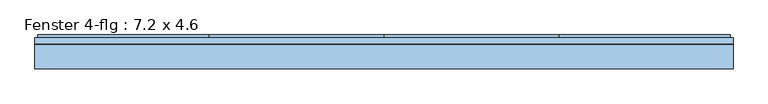
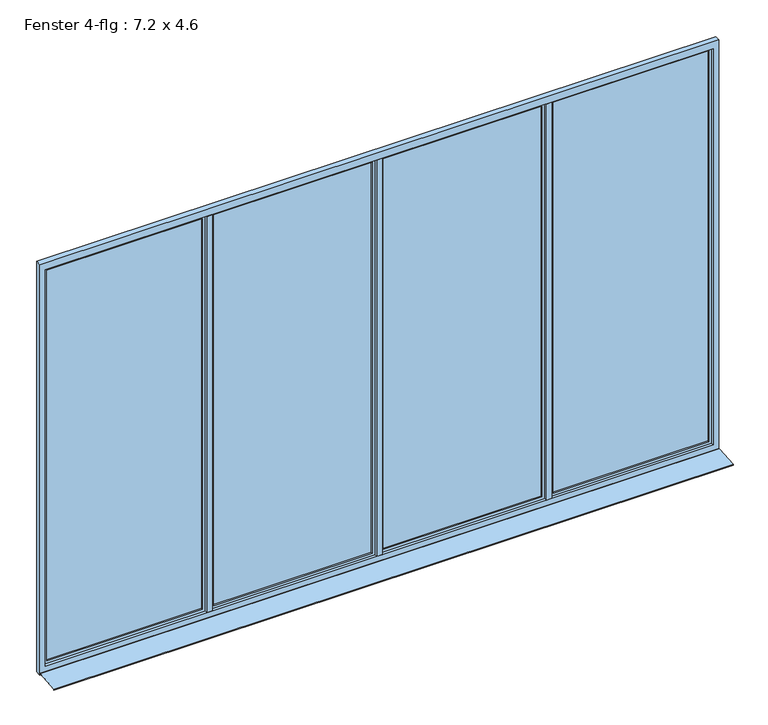
"""IFC4 building model written with IfcOpenShell, lengths in millimetres: window geometry, Fenster 4-flg : 7.2 x 4.6."""

import ifcopenshell
import ifcopenshell.guid

model = None  # the IFC model being written
_history = None  # IfcOwnerHistory: only IFC2X3 demands one
_inside = {}  # id of a spatial element -> (the spatial element, [elements in it])
_under = {}  # id of a project, library or spatial element -> (it, [spatial elements below it])
_declared = {}  # id of a project -> (the project, [libraries it declares])
_typed = {}  # id of a type object -> (the type object, [elements of that type])
_made_of = {}  # id of a material, layer set ... -> (it, [elements and type objects made of it])


def new_model(schema):
    """Start an empty IFC model of exactly this schema.

    Asked for "IFC4X3", IfcOpenShell would pick the latest addendum, in which some entities
    have other attributes; the version numbers below select the first issue.
    IFC2X3 requires an IfcOwnerHistory on every rooted entity: one is made here for all.
    """
    global model, _history
    if schema == "IFC4X3":
        model = ifcopenshell.file(schema_version=(4, 3, 0, 0))
    else:
        model = ifcopenshell.file(schema=schema)
    _inside.clear()
    _under.clear()
    _declared.clear()
    _typed.clear()
    _made_of.clear()
    _history = None
    if model.schema == "IFC2X3":
        org = make("IfcOrganization", Name="unknown")
        user = make(
            "IfcPersonAndOrganization",
            ThePerson=make("IfcPerson", FamilyName="unknown"),
            TheOrganization=org,
        )
        app = make(
            "IfcApplication",
            ApplicationDeveloper=org,
            Version="unknown",
            ApplicationFullName="unknown",
            ApplicationIdentifier="unknown",
        )
        _history = make(
            "IfcOwnerHistory",
            OwningUser=user,
            OwningApplication=app,
            ChangeAction="ADDED",
            CreationDate=0,
        )
    return model


def make(cls, **values):
    """One entity of the class cls with the attributes given. An attribute that is None is left unset."""
    return model.create_entity(
        cls, **{name: value for name, value in values.items() if value is not None}
    )


def rooted(cls, **values):
    """An entity with a GlobalId (a new one), such as an element, a storey or a relation."""
    return make(cls, GlobalId=ifcopenshell.guid.new(), OwnerHistory=_history, **values)


def si_unit(unit_type, name, prefix=None):
    """IfcSIUnit, for example si_unit("LENGTHUNIT", "METRE", prefix="MILLI")."""
    return make("IfcSIUnit", UnitType=unit_type, Prefix=prefix, Name=name)


def assignment(units):
    """IfcUnitAssignment: the units of a project."""
    return None if units is None else make("IfcUnitAssignment", Units=units)


def point(xyz):
    """IfcCartesianPoint."""
    return None if xyz is None else make("IfcCartesianPoint", Coordinates=xyz)


def direction(xyz):
    """IfcDirection."""
    return None if xyz is None else make("IfcDirection", DirectionRatios=xyz)


def frame(location, z_axis=None, x_axis=None):
    """IfcAxis2Placement3D, a coordinate frame: its origin and axes. An axis left out is left unset."""
    return make(
        "IfcAxis2Placement3D",
        Location=point(location),
        Axis=direction(z_axis),
        RefDirection=direction(x_axis),
    )


def origin():
    """The frame at (0, 0, 0) with its axes left unset."""
    return frame((0.0, 0.0, 0.0))


def place(relative_to, where):
    """IfcLocalPlacement: puts the frame where relative to a parent placement (None: the world)."""
    return make(
        "IfcLocalPlacement", PlacementRelTo=relative_to, RelativePlacement=where
    )


def context(
    kind, dimensions, precision=None, world=None, true_north=None, identifier=None
):
    """IfcGeometricRepresentationContext, for example the 3D "Model" context."""
    return make(
        "IfcGeometricRepresentationContext",
        ContextIdentifier=identifier,
        ContextType=kind,
        CoordinateSpaceDimension=dimensions,
        Precision=precision,
        WorldCoordinateSystem=world,
        TrueNorth=true_north,
    )


def project(units=None, contexts=None):
    """IfcProject with its units and contexts."""
    return rooted(
        "IfcProject",
        Name="project",
        RepresentationContexts=contexts,
        UnitsInContext=assignment(units),
    )


def spatial(cls, under=None, at=None, **own):
    """A site, building, storey or space (cls), placed at a placement, below another one or the project."""
    s = rooted(cls, ObjectPlacement=at, **own)
    if under is not None:
        _under.setdefault(under.id(), (under, []))[1].append(s)
    return s


def polyline(points):
    """IfcPolyline through the points."""
    return make("IfcPolyline", Points=[point(p) for p in points])


def outline(outer, holes=None, kind="AREA"):
    """IfcArbitraryClosedProfileDef: a profile drawn as a closed curve; with holes, ...WithVoids."""
    if holes is None:
        return make("IfcArbitraryClosedProfileDef", ProfileType=kind, OuterCurve=outer)
    return make(
        "IfcArbitraryProfileDefWithVoids",
        ProfileType=kind,
        OuterCurve=outer,
        InnerCurves=holes,
    )


def extrude(swept, where, along, depth):
    """IfcExtrudedAreaSolid: the profile swept, set in the frame where, extruded along a direction by depth."""
    return make(
        "IfcExtrudedAreaSolid",
        SweptArea=swept,
        Position=where,
        ExtrudedDirection=direction(along),
        Depth=depth,
    )


def faces_of(points, faces, orient=None, outer=None):
    """IfcFace entities. A face is a list of loops; a loop is a list of indices into points, from 0.

    orient and outer hold one flag for each loop. By default every Orientation is true, the
    first loop of a face is its IfcFaceOuterBound and the others are IfcFaceBound.
    """
    made = []
    for i, loops in enumerate(faces):
        bounds = []
        for j, loop in enumerate(loops):
            is_outer = j == 0 if outer is None else outer[i][j]
            bounds.append(
                make(
                    "IfcFaceOuterBound" if is_outer else "IfcFaceBound",
                    Bound=make("IfcPolyLoop", Polygon=[points[k] for k in loop]),
                    Orientation=True if orient is None else orient[i][j],
                )
            )
        made.append(make("IfcFace", Bounds=bounds))
    return made


def faceted_brep(points, faces, orient=None, outer=None, voids=None):
    """IfcFacetedBrep: a solid bounded by flat faces; with voids (closed shells), ...WithVoids."""
    shared = [point(p) for p in points]
    hull = make("IfcClosedShell", CfsFaces=faces_of(shared, faces, orient, outer))
    if voids is None:
        return make("IfcFacetedBrep", Outer=hull)
    return make(
        "IfcFacetedBrepWithVoids",
        Outer=hull,
        Voids=[
            make(cls, CfsFaces=faces_of(shared, fs, o, b)) for cls, fs, o, b in voids
        ],
    )


def shape(context_of_items, identifier, shape_type, items):
    """IfcShapeRepresentation: the items that make up one representation, for example the "Body"."""
    return make(
        "IfcShapeRepresentation",
        ContextOfItems=context_of_items,
        RepresentationIdentifier=identifier,
        RepresentationType=shape_type,
        Items=items,
    )


def source(mapping_origin, context_of_items, identifier, shape_type, items):
    """IfcRepresentationMap: a shape defined once, which mapped items show again and again."""
    return make(
        "IfcRepresentationMap",
        MappingOrigin=mapping_origin,
        MappedRepresentation=shape(context_of_items, identifier, shape_type, items),
    )


def transform(
    local_origin,
    x_axis=None,
    y_axis=None,
    z_axis=None,
    scale=None,
    scale2=None,
    scale3=None,
    uniform=True,
):
    """IfcCartesianTransformationOperator3D, or its non-uniform kind. x_axis, y_axis, z_axis: its Axis1, 2, 3."""
    if uniform:
        return make(
            "IfcCartesianTransformationOperator3D",
            Axis1=direction(x_axis),
            Axis2=direction(y_axis),
            LocalOrigin=point(local_origin),
            Scale=scale,
            Axis3=direction(z_axis),
        )
    return make(
        "IfcCartesianTransformationOperator3DnonUniform",
        Axis1=direction(x_axis),
        Axis2=direction(y_axis),
        LocalOrigin=point(local_origin),
        Scale=scale,
        Axis3=direction(z_axis),
        Scale2=scale2,
        Scale3=scale3,
    )


def mapped(mapping_source, mapping_target):
    """IfcMappedItem: shows the shape of a source again, moved by a transform."""
    return make(
        "IfcMappedItem", MappingSource=mapping_source, MappingTarget=mapping_target
    )


def made_of(thing, what):
    """Note that an element or type object is made of a material, layer set ...; save() writes the relation."""
    if what is not None:
        _made_of.setdefault(what.id(), (what, []))[1].append(thing)
    return thing


def element(
    cls,
    number,
    at=None,
    inside=None,
    cuts=None,
    type_object=None,
    material=None,
    context=None,
    identifier="Body",
    shape_type=None,
    held_by="IfcProductDefinitionShape",
    body=None,
    shapes=None,
    **own,
):
    """One element of the class cls, such as IfcWall. Its Tag is "e" and its number.

    at: its placement. inside: the storey or other place that contains it. cuts: it is an
    opening in that element (IfcRelVoidsElement). A single representation is given by context,
    identifier, shape_type and body (its items); several are given by shapes. held_by: the class
    of the entity that holds the representations. save() writes the other relations.
    """
    e = rooted(cls, Tag="e%d" % number, ObjectPlacement=at, **own)
    if body is not None:
        shapes = [shape(context, identifier, shape_type, body)]
    if shapes is not None:
        e.Representation = make(held_by, Representations=shapes)
    if inside is not None:
        _inside.setdefault(inside.id(), (inside, []))[1].append(e)
    if cuts is not None:
        rooted(
            "IfcRelVoidsElement", RelatingBuildingElement=cuts, RelatedOpeningElement=e
        )
    if type_object is not None:
        _typed.setdefault(type_object.id(), (type_object, []))[1].append(e)
    return made_of(e, material)


def aggregate(whole, parts):
    """IfcRelAggregates: a whole, such as a stair, and the parts it consists of."""
    return rooted("IfcRelAggregates", RelatingObject=whole, RelatedObjects=parts)


def save(model, path):
    """Write the relations noted so far, then the file.

    IfcRelAggregates (storeys below a building ...), IfcRelContainedInSpatialStructure (elements
    in a storey), IfcRelDefinesByType, IfcRelAssociatesMaterial and IfcRelDeclares: one each for
    every whole, place, type object, material and project.
    """
    for whole, parts in _under.values():
        aggregate(whole, parts)
    for where, things in _inside.values():
        rooted(
            "IfcRelContainedInSpatialStructure",
            RelatedElements=things,
            RelatingStructure=where,
        )
    for kind, things in _typed.values():
        rooted("IfcRelDefinesByType", RelatedObjects=things, RelatingType=kind)
    for what, things in _made_of.values():
        rooted("IfcRelAssociatesMaterial", RelatedObjects=things, RelatingMaterial=what)
    for by, libraries in _declared.values():
        rooted("IfcRelDeclares", RelatingContext=by, RelatedDefinitions=libraries)
    model.write(path)


def fenster_4_flg_7_2_x_4_6_69958212(model_context):
    return source(origin(), model_context, "Body", "SolidModel", [
        extrude(outline(polyline([(4300.0, -80.0), (4240.0, -80.0), (4240.0, -20.0), (4300.0, -20.0), (4300.0, -80.0)])), frame((0.0, 0.0, 1080.0), z_axis=(0.0, 0.0, 1.0), x_axis=(1.0, 0.0, 0.0)), (0.0, 0.0, 1.0), 4440.0),
        extrude(outline(polyline([(2500.0, -80.0), (2440.0, -80.0), (2440.0, -20.0), (2500.0, -20.0), (2500.0, -80.0)])), frame((0.0, 0.0, 1080.0), z_axis=(0.0, 0.0, 1.0), x_axis=(1.0, 0.0, 0.0)), (0.0, 0.0, 1.0), 4440.0),
        extrude(outline(polyline([(700.0, -80.0), (640.0, -80.0), (640.0, -20.0), (700.0, -20.0), (700.0, -80.0)])), frame((0.0, 0.0, 1080.0), z_axis=(0.0, 0.0, 1.0), x_axis=(1.0, 0.0, 0.0)), (0.0, 0.0, 1.0), 4440.0),
        extrude(outline(polyline([(5600.0, 6070.0), (5600.0, -1130.0), (1000.0, -1130.0), (1000.0, 6070.0), (5600.0, 6070.0)]), holes=[polyline([(5520.0, 6010.0), (1080.0, 6010.0), (1080.0, -1070.0), (5520.0, -1070.0), (5520.0, 6010.0)])]), frame((0.0, -80.0, 0.0), z_axis=(0.0, 1.0, 0.0), x_axis=(0.0, 0.0, 1.0)), (0.0, 0.0, 1.0), 60.0),
        faceted_brep([(4270.0, -20.0, 5550.0), (4270.0, -20.0, 1050.0), (4270.0, 10.0, 1050.0), (4270.0, 10.0, 5550.0), (2470.0, 10.0, 1050.0), (2470.0, 10.0, 5550.0), (4210.0, 10.0, 1110.0), (4210.0, 10.0, 5490.0), (2530.0, 10.0, 5490.0), (2530.0, 10.0, 1110.0), (2470.0, -20.0, 1050.0), (2470.0, -20.0, 5550.0), (4240.0, -20.0, 5520.0), (4240.0, -20.0, 1080.0), (2500.0, -20.0, 1080.0), (2500.0, -20.0, 5520.0), (4240.0, -50.0, 5520.0), (4240.0, -50.0, 1080.0), (2500.0, -50.0, 1080.0), (2500.0, -50.0, 5520.0), (4210.0, -50.0, 5490.0), (4210.0, -50.0, 1110.0), (2530.0, -50.0, 1110.0), (2530.0, -50.0, 5490.0)], [[[0, 1, 2, 3]], [[3, 2, 4, 5], [6, 7, 8, 9]], [[1, 10, 4, 2]], [[1, 0, 11, 10], [12, 13, 14, 15]], [[16, 17, 13, 12]], [[17, 18, 14, 13]], [[17, 16, 19, 18], [20, 21, 22, 23]], [[7, 6, 21, 20]], [[6, 9, 22, 21]], [[10, 11, 5, 4]], [[18, 19, 15, 14]], [[9, 8, 23, 22]], [[11, 0, 3, 5]], [[19, 16, 12, 15]], [[8, 7, 20, 23]]]),
        faceted_brep([(2470.0, -20.0, 5550.0), (2470.0, -20.0, 1050.0), (2470.0, 10.0, 1050.0), (2470.0, 10.0, 5550.0), (670.0, 10.0, 1050.0), (670.0, 10.0, 5550.0), (2410.0, 10.0, 1110.0), (2410.0, 10.0, 5490.0), (730.0, 10.0, 5490.0), (730.0, 10.0, 1110.0), (670.0, -20.0, 1050.0), (670.0, -20.0, 5550.0), (2440.0, -20.0, 5520.0), (2440.0, -20.0, 1080.0), (700.0, -20.0, 1080.0), (700.0, -20.0, 5520.0), (2440.0, -50.0, 5520.0), (2440.0, -50.0, 1080.0), (700.0, -50.0, 1080.0), (700.0, -50.0, 5520.0), (2410.0, -50.0, 5490.0), (2410.0, -50.0, 1110.0), (730.0, -50.0, 1110.0), (730.0, -50.0, 5490.0)], [[[0, 1, 2, 3]], [[3, 2, 4, 5], [6, 7, 8, 9]], [[1, 10, 4, 2]], [[1, 0, 11, 10], [12, 13, 14, 15]], [[16, 17, 13, 12]], [[17, 18, 14, 13]], [[17, 16, 19, 18], [20, 21, 22, 23]], [[7, 6, 21, 20]], [[6, 9, 22, 21]], [[10, 11, 5, 4]], [[18, 19, 15, 14]], [[9, 8, 23, 22]], [[11, 0, 3, 5]], [[19, 16, 12, 15]], [[8, 7, 20, 23]]]),
        faceted_brep([(670.0, -20.0, 5550.0), (670.0, -20.0, 1050.0), (670.0, 10.0, 1050.0), (670.0, 10.0, 5550.0), (-1100.0, 10.0, 1050.0), (-1100.0, 10.0, 5550.0), (610.0, 10.0, 1110.0), (610.0, 10.0, 5490.0), (-1040.0, 10.0, 5490.0), (-1040.0, 10.0, 1110.0), (-1100.0, -20.0, 1050.0), (-1100.0, -20.0, 5550.0), (640.0, -20.0, 5520.0), (640.0, -20.0, 1080.0), (-1070.0, -20.0, 1080.0), (-1070.0, -20.0, 5520.0), (640.0, -50.0, 5520.0), (640.0, -50.0, 1080.0), (-1070.0, -50.0, 1080.0), (-1070.0, -50.0, 5520.0), (610.0, -50.0, 5490.0), (610.0, -50.0, 1110.0), (-1040.0, -50.0, 1110.0), (-1040.0, -50.0, 5490.0)], [[[0, 1, 2, 3]], [[3, 2, 4, 5], [6, 7, 8, 9]], [[1, 10, 4, 2]], [[1, 0, 11, 10], [12, 13, 14, 15]], [[16, 17, 13, 12]], [[17, 18, 14, 13]], [[17, 16, 19, 18], [20, 21, 22, 23]], [[7, 6, 21, 20]], [[6, 9, 22, 21]], [[10, 11, 5, 4]], [[18, 19, 15, 14]], [[9, 8, 23, 22]], [[11, 0, 3, 5]], [[19, 16, 12, 15]], [[8, 7, 20, 23]]]),
        faceted_brep([(6040.0, -20.0, 5550.0), (6040.0, -20.0, 1050.0), (6040.0, 10.0, 1050.0), (6040.0, 10.0, 5550.0), (4270.0, 10.0, 1050.0), (4270.0, 10.0, 5550.0), (5980.0, 10.0, 1110.0), (5980.0, 10.0, 5490.0), (4330.0, 10.0, 5490.0), (4330.0, 10.0, 1110.0), (4270.0, -20.0, 1050.0), (4270.0, -20.0, 5550.0), (6010.0, -20.0, 5520.0), (6010.0, -20.0, 1080.0), (4300.0, -20.0, 1080.0), (4300.0, -20.0, 5520.0), (6010.0, -50.0, 5520.0), (6010.0, -50.0, 1080.0), (4300.0, -50.0, 1080.0), (4300.0, -50.0, 5520.0), (5980.0, -50.0, 5490.0), (5980.0, -50.0, 1110.0), (4330.0, -50.0, 1110.0), (4330.0, -50.0, 5490.0)], [[[0, 1, 2, 3]], [[3, 2, 4, 5], [6, 7, 8, 9]], [[1, 10, 4, 2]], [[1, 0, 11, 10], [12, 13, 14, 15]], [[16, 17, 13, 12]], [[17, 18, 14, 13]], [[17, 16, 19, 18], [20, 21, 22, 23]], [[7, 6, 21, 20]], [[6, 9, 22, 21]], [[10, 11, 5, 4]], [[18, 19, 15, 14]], [[9, 8, 23, 22]], [[11, 0, 3, 5]], [[19, 16, 12, 15]], [[8, 7, 20, 23]]]),
        extrude(outline(polyline([(-90.0221543, 1020.0), (-80.0, 1020.0), (-80.0, 1018.0), (-89.8240723, 1018.0), (-338.0, 998.3604634), (-338.0, 990.0), (-340.0, 990.0), (-340.0, 1000.0), (-90.0221543, 1020.0)])), frame((-1130.0, 0.0, 0.0), z_axis=(1.0, 0.0, 0.0), x_axis=(0.0, 1.0, 0.0)), (0.0, 0.0, 1.0), 7200.0),
        extrude(outline(polyline([(610.0, -5.0), (610.0, -35.0), (-1040.0, -35.0), (-1040.0, -5.0), (610.0, -5.0)])), frame((0.0, 0.0, 1110.0), z_axis=(0.0, 0.0, 1.0), x_axis=(1.0, 0.0, 0.0)), (0.0, 0.0, 1.0), 4380.0),
        extrude(outline(polyline([(2410.0, -5.0), (2410.0, -35.0), (730.0, -35.0), (730.0, -5.0), (2410.0, -5.0)])), frame((0.0, 0.0, 1110.0), z_axis=(0.0, 0.0, 1.0), x_axis=(1.0, 0.0, 0.0)), (0.0, 0.0, 1.0), 4380.0),
        extrude(outline(polyline([(4210.0, -5.0), (4210.0, -35.0), (2530.0, -35.0), (2530.0, -5.0), (4210.0, -5.0)])), frame((0.0, 0.0, 1110.0), z_axis=(0.0, 0.0, 1.0), x_axis=(1.0, 0.0, 0.0)), (0.0, 0.0, 1.0), 4380.0),
        extrude(outline(polyline([(5980.0, -5.0), (5980.0, -35.0), (4330.0, -35.0), (4330.0, -5.0), (5980.0, -5.0)])), frame((0.0, 0.0, 1110.0), z_axis=(0.0, 0.0, 1.0), x_axis=(1.0, 0.0, 0.0)), (0.0, 0.0, 1.0), 4380.0),
    ])


if __name__ == "__main__":
    model = new_model("IFC4")
    model_context = context("Model", 3, world=origin())
    ifc_project = project(units=[si_unit("LENGTHUNIT", "METRE", prefix="MILLI")], contexts=[model_context])
    site = spatial("IfcSite", under=ifc_project)
    building = spatial("IfcBuilding", under=site)
    placement = place(None, origin())
    fenster_4_flg_7_2_x_4_6_shape = fenster_4_flg_7_2_x_4_6_69958212(model_context)
    element("IfcWindow", 1, ObjectType="Fenster 4-flg : 7.2 x 4.6", at=placement, inside=building, context=model_context, shape_type="MappedRepresentation", body=[
        mapped(fenster_4_flg_7_2_x_4_6_shape, transform((0.0, 0.0, 0.0), x_axis=(1.0, 0.0, 0.0), y_axis=(0.0, 1.0, 0.0), z_axis=(0.0, 0.0, 1.0))),
    ])
    save(model, "model.ifc")

# Revit data of these elements
# Type "Fenster 4-flg : 7.2 x 4.6"
#   Type Mark = "55"
#   Operation = "UserDefined"
#   Keynote = "16.05.01"
#   Visual Light Transmittance = 0.9
#   Solar Heat Gain Coefficient = 0.78
#   Rough Height = 4.600 m
#   Rough Width = 7.200 m
#   Heat Transfer Coefficient (U) = 3.6886 W/(m²·K)
#   Rahmentiefe = 0.060 m
#   Breite unterer Rahmen = 0.080 m
#   Breite oberer  Rahmen = 0.080 m
#   Rahmenbreite = 0.060 m
#   Height = 4.600 m
#   Tiefe Flügel = 0.060 m
#   Flügelbreite = 0.060 m
#   Einbautiefe (von außen) [instance default] = 0.080 m
#   Width = 7.200 m
#   Bild = none
#   Glas = Fenster - Glas
#   Fensterflügel = Fenster - Kunststoff weiß
#   Innere Fensterbank = Fenster - Holz 1
#   Äußere Fensterbank = Fenster - Kunststoff weiß
#   Construction Type Id = ""
#   Wall Closure = (empty or 0)
#   Analytic Construction = (empty or 0)
# Element 1 (IfcWindow, "Fenster 4-flg : 7.2 x 4.6")
#   Einbautiefe (von außen) = 0.230 m
#   Materials on its faces: "Fenster - Kunststoff weiß", "Kunststoff - Weiß", "Fenster - Glas"
# Materials
#   "Fenster - Glas": class "Glas", colour RGB 128 128 255, transparency 0.75, Cost = 0
#   "Fenster - Kunststoff weiß": class "Kunststoff", colour RGB 249 249 249, transparency 0, Cost = 0
#   "Fenster - Holz 1": class "Holz", colour RGB 216 135 75, transparency 0, Cost = 0
#   "Kunststoff - Weiß": class "Kunststoff", colour RGB 249 249 249, transparency 0, Cost = 0
